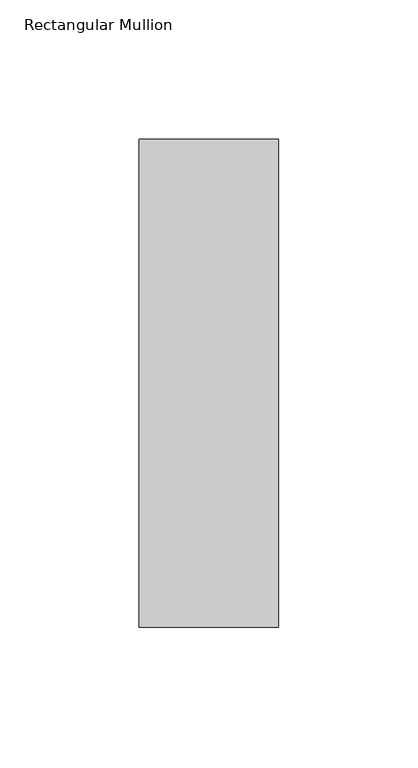
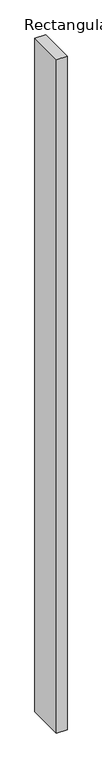
"""IFC4 building model written with IfcOpenShell, lengths in millimetres: member geometry, Rectangular Mullion : WWm-50x175-50mmOffset."""

import ifcopenshell
import ifcopenshell.guid

model = None  # the IFC model being written
_history = None  # IfcOwnerHistory: only IFC2X3 demands one
_inside = {}  # id of a spatial element -> (the spatial element, [elements in it])
_under = {}  # id of a project, library or spatial element -> (it, [spatial elements below it])
_declared = {}  # id of a project -> (the project, [libraries it declares])
_typed = {}  # id of a type object -> (the type object, [elements of that type])
_made_of = {}  # id of a material, layer set ... -> (it, [elements and type objects made of it])


def new_model(schema):
    """Start an empty IFC model of exactly this schema.

    Asked for "IFC4X3", IfcOpenShell would pick the latest addendum, in which some entities
    have other attributes; the version numbers below select the first issue.
    IFC2X3 requires an IfcOwnerHistory on every rooted entity: one is made here for all.
    """
    global model, _history
    if schema == "IFC4X3":
        model = ifcopenshell.file(schema_version=(4, 3, 0, 0))
    else:
        model = ifcopenshell.file(schema=schema)
    _inside.clear()
    _under.clear()
    _declared.clear()
    _typed.clear()
    _made_of.clear()
    _history = None
    if model.schema == "IFC2X3":
        org = make("IfcOrganization", Name="unknown")
        user = make(
            "IfcPersonAndOrganization",
            ThePerson=make("IfcPerson", FamilyName="unknown"),
            TheOrganization=org,
        )
        app = make(
            "IfcApplication",
            ApplicationDeveloper=org,
            Version="unknown",
            ApplicationFullName="unknown",
            ApplicationIdentifier="unknown",
        )
        _history = make(
            "IfcOwnerHistory",
            OwningUser=user,
            OwningApplication=app,
            ChangeAction="ADDED",
            CreationDate=0,
        )
    return model


def make(cls, **values):
    """One entity of the class cls with the attributes given. An attribute that is None is left unset."""
    return model.create_entity(
        cls, **{name: value for name, value in values.items() if value is not None}
    )


def rooted(cls, **values):
    """An entity with a GlobalId (a new one), such as an element, a storey or a relation."""
    return make(cls, GlobalId=ifcopenshell.guid.new(), OwnerHistory=_history, **values)


def si_unit(unit_type, name, prefix=None):
    """IfcSIUnit, for example si_unit("LENGTHUNIT", "METRE", prefix="MILLI")."""
    return make("IfcSIUnit", UnitType=unit_type, Prefix=prefix, Name=name)


def assignment(units):
    """IfcUnitAssignment: the units of a project."""
    return None if units is None else make("IfcUnitAssignment", Units=units)


def point(xyz):
    """IfcCartesianPoint."""
    return None if xyz is None else make("IfcCartesianPoint", Coordinates=xyz)


def direction(xyz):
    """IfcDirection."""
    return None if xyz is None else make("IfcDirection", DirectionRatios=xyz)


def frame(location, z_axis=None, x_axis=None):
    """IfcAxis2Placement3D, a coordinate frame: its origin and axes. An axis left out is left unset."""
    return make(
        "IfcAxis2Placement3D",
        Location=point(location),
        Axis=direction(z_axis),
        RefDirection=direction(x_axis),
    )


def origin():
    """The frame at (0, 0, 0) with its axes left unset."""
    return frame((0.0, 0.0, 0.0))


def place(relative_to, where):
    """IfcLocalPlacement: puts the frame where relative to a parent placement (None: the world)."""
    return make(
        "IfcLocalPlacement", PlacementRelTo=relative_to, RelativePlacement=where
    )


def context(
    kind, dimensions, precision=None, world=None, true_north=None, identifier=None
):
    """IfcGeometricRepresentationContext, for example the 3D "Model" context."""
    return make(
        "IfcGeometricRepresentationContext",
        ContextIdentifier=identifier,
        ContextType=kind,
        CoordinateSpaceDimension=dimensions,
        Precision=precision,
        WorldCoordinateSystem=world,
        TrueNorth=true_north,
    )


def project(units=None, contexts=None):
    """IfcProject with its units and contexts."""
    return rooted(
        "IfcProject",
        Name="project",
        RepresentationContexts=contexts,
        UnitsInContext=assignment(units),
    )


def spatial(cls, under=None, at=None, **own):
    """A site, building, storey or space (cls), placed at a placement, below another one or the project."""
    s = rooted(cls, ObjectPlacement=at, **own)
    if under is not None:
        _under.setdefault(under.id(), (under, []))[1].append(s)
    return s


def polyline(points):
    """IfcPolyline through the points."""
    return make("IfcPolyline", Points=[point(p) for p in points])


def outline(outer, holes=None, kind="AREA"):
    """IfcArbitraryClosedProfileDef: a profile drawn as a closed curve; with holes, ...WithVoids."""
    if holes is None:
        return make("IfcArbitraryClosedProfileDef", ProfileType=kind, OuterCurve=outer)
    return make(
        "IfcArbitraryProfileDefWithVoids",
        ProfileType=kind,
        OuterCurve=outer,
        InnerCurves=holes,
    )


def extrude(swept, where, along, depth):
    """IfcExtrudedAreaSolid: the profile swept, set in the frame where, extruded along a direction by depth."""
    return make(
        "IfcExtrudedAreaSolid",
        SweptArea=swept,
        Position=where,
        ExtrudedDirection=direction(along),
        Depth=depth,
    )


def shape(context_of_items, identifier, shape_type, items):
    """IfcShapeRepresentation: the items that make up one representation, for example the "Body"."""
    return make(
        "IfcShapeRepresentation",
        ContextOfItems=context_of_items,
        RepresentationIdentifier=identifier,
        RepresentationType=shape_type,
        Items=items,
    )


def source(mapping_origin, context_of_items, identifier, shape_type, items):
    """IfcRepresentationMap: a shape defined once, which mapped items show again and again."""
    return make(
        "IfcRepresentationMap",
        MappingOrigin=mapping_origin,
        MappedRepresentation=shape(context_of_items, identifier, shape_type, items),
    )


def transform(
    local_origin,
    x_axis=None,
    y_axis=None,
    z_axis=None,
    scale=None,
    scale2=None,
    scale3=None,
    uniform=True,
):
    """IfcCartesianTransformationOperator3D, or its non-uniform kind. x_axis, y_axis, z_axis: its Axis1, 2, 3."""
    if uniform:
        return make(
            "IfcCartesianTransformationOperator3D",
            Axis1=direction(x_axis),
            Axis2=direction(y_axis),
            LocalOrigin=point(local_origin),
            Scale=scale,
            Axis3=direction(z_axis),
        )
    return make(
        "IfcCartesianTransformationOperator3DnonUniform",
        Axis1=direction(x_axis),
        Axis2=direction(y_axis),
        LocalOrigin=point(local_origin),
        Scale=scale,
        Axis3=direction(z_axis),
        Scale2=scale2,
        Scale3=scale3,
    )


def mapped(mapping_source, mapping_target):
    """IfcMappedItem: shows the shape of a source again, moved by a transform."""
    return make(
        "IfcMappedItem", MappingSource=mapping_source, MappingTarget=mapping_target
    )


def made_of(thing, what):
    """Note that an element or type object is made of a material, layer set ...; save() writes the relation."""
    if what is not None:
        _made_of.setdefault(what.id(), (what, []))[1].append(thing)
    return thing


def element(
    cls,
    number,
    at=None,
    inside=None,
    cuts=None,
    type_object=None,
    material=None,
    context=None,
    identifier="Body",
    shape_type=None,
    held_by="IfcProductDefinitionShape",
    body=None,
    shapes=None,
    **own,
):
    """One element of the class cls, such as IfcWall. Its Tag is "e" and its number.

    at: its placement. inside: the storey or other place that contains it. cuts: it is an
    opening in that element (IfcRelVoidsElement). A single representation is given by context,
    identifier, shape_type and body (its items); several are given by shapes. held_by: the class
    of the entity that holds the representations. save() writes the other relations.
    """
    e = rooted(cls, Tag="e%d" % number, ObjectPlacement=at, **own)
    if body is not None:
        shapes = [shape(context, identifier, shape_type, body)]
    if shapes is not None:
        e.Representation = make(held_by, Representations=shapes)
    if inside is not None:
        _inside.setdefault(inside.id(), (inside, []))[1].append(e)
    if cuts is not None:
        rooted(
            "IfcRelVoidsElement", RelatingBuildingElement=cuts, RelatedOpeningElement=e
        )
    if type_object is not None:
        _typed.setdefault(type_object.id(), (type_object, []))[1].append(e)
    return made_of(e, material)


def aggregate(whole, parts):
    """IfcRelAggregates: a whole, such as a stair, and the parts it consists of."""
    return rooted("IfcRelAggregates", RelatingObject=whole, RelatedObjects=parts)


def save(model, path):
    """Write the relations noted so far, then the file.

    IfcRelAggregates (storeys below a building ...), IfcRelContainedInSpatialStructure (elements
    in a storey), IfcRelDefinesByType, IfcRelAssociatesMaterial and IfcRelDeclares: one each for
    every whole, place, type object, material and project.
    """
    for whole, parts in _under.values():
        aggregate(whole, parts)
    for where, things in _inside.values():
        rooted(
            "IfcRelContainedInSpatialStructure",
            RelatedElements=things,
            RelatingStructure=where,
        )
    for kind, things in _typed.values():
        rooted("IfcRelDefinesByType", RelatedObjects=things, RelatingType=kind)
    for what, things in _made_of.values():
        rooted("IfcRelAssociatesMaterial", RelatedObjects=things, RelatingMaterial=what)
    for by, libraries in _declared.values():
        rooted("IfcRelDeclares", RelatingContext=by, RelatedDefinitions=libraries)
    model.write(path)


def rectangular_mullion_7b5d3532(model_context):
    return source(origin(), model_context, "Body", "SweptSolid", [
        extrude(outline(polyline([(25.0, 87.5), (25.0, -87.5), (-25.0, -87.5), (-25.0, 87.5), (25.0, 87.5)])), frame((0.0, 0.0, -3350.0), z_axis=(0.0, 0.0, 1.0), x_axis=(1.0, 0.0, 0.0)), (0.0, 0.0, 1.0), 3350.0),
    ])


if __name__ == "__main__":
    model = new_model("IFC4")
    model_context = context("Model", 3, world=origin())
    ifc_project = project(units=[si_unit("LENGTHUNIT", "METRE", prefix="MILLI")], contexts=[model_context])
    site = spatial("IfcSite", under=ifc_project)
    building = spatial("IfcBuilding", under=site)
    placement = place(None, origin())
    rectangular_mullion_shape = rectangular_mullion_7b5d3532(model_context)
    element("IfcMember", 1, ObjectType="Rectangular Mullion : WWm-50x175-50mmOffset", at=placement, inside=building, context=model_context, shape_type="MappedRepresentation", body=[
        mapped(rectangular_mullion_shape, transform((0.0, 0.0, 0.0), x_axis=(1.0, 0.0, 0.0), y_axis=(0.0, 1.0, 0.0), z_axis=(0.0, 0.0, 1.0))),
    ])
    save(model, "model.ifc")

# Revit data of these elements
# Type "Rectangular Mullion : WWm-50x175-50mmOffset"
#   built-in parameter 1007304 = 0.574147 (stored number, unit not read)
#   built-in parameter 1007301 = 0.082021 (stored number, unit not read)
#   built-in parameter 1007300 = 0.082021 (stored number, unit not read)
# Element 1 (IfcMember, "Rectangular Mullion : WWm-50x175-50mmOffset")
#   Materials on its faces: "WW-EC-RGB-Mullion"
# Materials
#   "WW-EC-RGB-Mullion": class "Generic", colour RGB 255 255 255, transparency 0, Comments = "If region requests black mullions, switch asset color to RGB 25-25-25", Description = "Generic Color", Cost = 0
